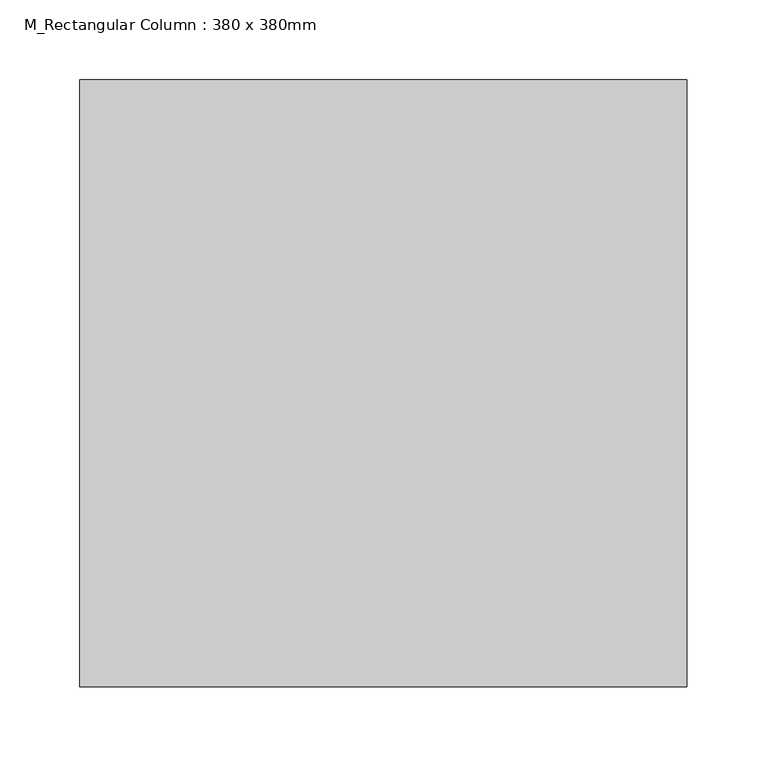
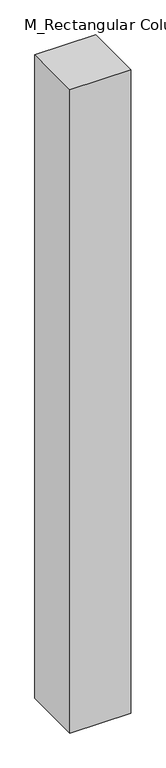
"""IFC4 building model written with IfcOpenShell, lengths in millimetres: column geometry, M_Rectangular Column : 380 x 380mm."""

from ifc_helpers import new_model, si_unit, frame, origin, place, context, project, spatial, polyline, outline, extrude, source, transform, mapped, element, save


def m_rectangular_column_380_x_380mm_f7aa0fc7(model_context):
    return source(origin(), model_context, "Body", "SweptSolid", [
        extrude(outline(polyline([(190.0, 190.0), (190.0, -190.0), (-190.0, -190.0), (-190.0, 190.0), (190.0, 190.0)])), frame((0.0, 0.0, 40.0), z_axis=(0.0, 0.0, 1.0), x_axis=(1.0, 0.0, 0.0)), (0.0, 0.0, 1.0), 4260.0),
    ])


if __name__ == "__main__":
    model = new_model("IFC4")
    model_context = context("Model", 3, world=origin())
    ifc_project = project(units=[si_unit("LENGTHUNIT", "METRE", prefix="MILLI")], contexts=[model_context])
    site = spatial("IfcSite", under=ifc_project)
    building = spatial("IfcBuilding", under=site)
    placement = place(None, origin())
    m_rectangular_column_380_x_380mm_shape = m_rectangular_column_380_x_380mm_f7aa0fc7(model_context)
    element("IfcColumn", 1, ObjectType="M_Rectangular Column : 380 x 380mm", at=placement, inside=building, context=model_context, shape_type="MappedRepresentation", body=[
        mapped(m_rectangular_column_380_x_380mm_shape, transform((0.0, 0.0, 0.0), x_axis=(1.0, 0.0, 0.0), y_axis=(0.0, 1.0, 0.0), z_axis=(0.0, 0.0, 1.0))),
    ])
    save(model, "model.ifc")

# Revit data of these elements
# Type "M_Rectangular Column : 380 x 380mm"
#   Depth = 38.0 cm
#   Offset Base = 0.0 cm
#   Offset Top = 0.0 cm
#   Width = 38.0 cm
#   Material = none
